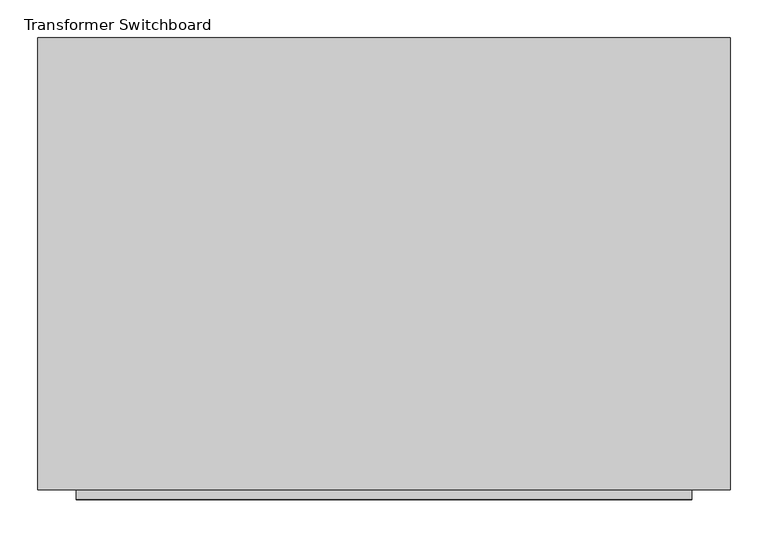
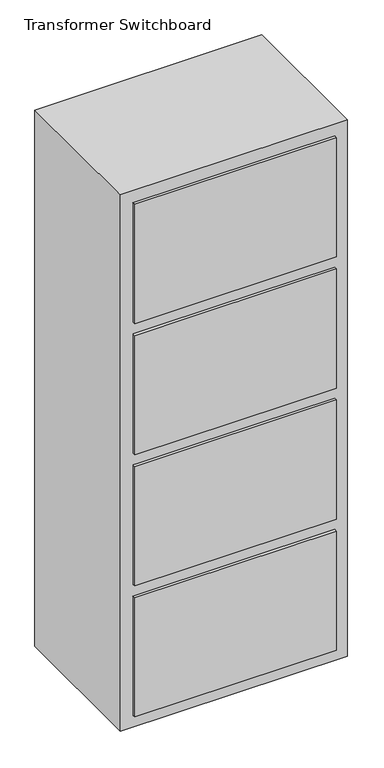
"""IFC4 building model written with IfcOpenShell, lengths in millimetres: proxy geometry, Transformer Switchboard."""

import ifcopenshell
import ifcopenshell.guid

model = None  # the IFC model being written
_history = None  # IfcOwnerHistory: only IFC2X3 demands one
_inside = {}  # id of a spatial element -> (the spatial element, [elements in it])
_under = {}  # id of a project, library or spatial element -> (it, [spatial elements below it])
_declared = {}  # id of a project -> (the project, [libraries it declares])
_typed = {}  # id of a type object -> (the type object, [elements of that type])
_made_of = {}  # id of a material, layer set ... -> (it, [elements and type objects made of it])


def new_model(schema):
    """Start an empty IFC model of exactly this schema.

    Asked for "IFC4X3", IfcOpenShell would pick the latest addendum, in which some entities
    have other attributes; the version numbers below select the first issue.
    IFC2X3 requires an IfcOwnerHistory on every rooted entity: one is made here for all.
    """
    global model, _history
    if schema == "IFC4X3":
        model = ifcopenshell.file(schema_version=(4, 3, 0, 0))
    else:
        model = ifcopenshell.file(schema=schema)
    _inside.clear()
    _under.clear()
    _declared.clear()
    _typed.clear()
    _made_of.clear()
    _history = None
    if model.schema == "IFC2X3":
        org = make("IfcOrganization", Name="unknown")
        user = make(
            "IfcPersonAndOrganization",
            ThePerson=make("IfcPerson", FamilyName="unknown"),
            TheOrganization=org,
        )
        app = make(
            "IfcApplication",
            ApplicationDeveloper=org,
            Version="unknown",
            ApplicationFullName="unknown",
            ApplicationIdentifier="unknown",
        )
        _history = make(
            "IfcOwnerHistory",
            OwningUser=user,
            OwningApplication=app,
            ChangeAction="ADDED",
            CreationDate=0,
        )
    return model


def make(cls, **values):
    """One entity of the class cls with the attributes given. An attribute that is None is left unset."""
    return model.create_entity(
        cls, **{name: value for name, value in values.items() if value is not None}
    )


def rooted(cls, **values):
    """An entity with a GlobalId (a new one), such as an element, a storey or a relation."""
    return make(cls, GlobalId=ifcopenshell.guid.new(), OwnerHistory=_history, **values)


def si_unit(unit_type, name, prefix=None):
    """IfcSIUnit, for example si_unit("LENGTHUNIT", "METRE", prefix="MILLI")."""
    return make("IfcSIUnit", UnitType=unit_type, Prefix=prefix, Name=name)


def assignment(units):
    """IfcUnitAssignment: the units of a project."""
    return None if units is None else make("IfcUnitAssignment", Units=units)


def point(xyz):
    """IfcCartesianPoint."""
    return None if xyz is None else make("IfcCartesianPoint", Coordinates=xyz)


def direction(xyz):
    """IfcDirection."""
    return None if xyz is None else make("IfcDirection", DirectionRatios=xyz)


def frame(location, z_axis=None, x_axis=None):
    """IfcAxis2Placement3D, a coordinate frame: its origin and axes. An axis left out is left unset."""
    return make(
        "IfcAxis2Placement3D",
        Location=point(location),
        Axis=direction(z_axis),
        RefDirection=direction(x_axis),
    )


def origin():
    """The frame at (0, 0, 0) with its axes left unset."""
    return frame((0.0, 0.0, 0.0))


def origin_with_axes():
    """The frame at (0, 0, 0) with the z axis (0, 0, 1) and the x axis (1, 0, 0) written out."""
    return frame((0.0, 0.0, 0.0), z_axis=(0.0, 0.0, 1.0), x_axis=(1.0, 0.0, 0.0))


def place(relative_to, where):
    """IfcLocalPlacement: puts the frame where relative to a parent placement (None: the world)."""
    return make(
        "IfcLocalPlacement", PlacementRelTo=relative_to, RelativePlacement=where
    )


def context(
    kind, dimensions, precision=None, world=None, true_north=None, identifier=None
):
    """IfcGeometricRepresentationContext, for example the 3D "Model" context."""
    return make(
        "IfcGeometricRepresentationContext",
        ContextIdentifier=identifier,
        ContextType=kind,
        CoordinateSpaceDimension=dimensions,
        Precision=precision,
        WorldCoordinateSystem=world,
        TrueNorth=true_north,
    )


def project(units=None, contexts=None):
    """IfcProject with its units and contexts."""
    return rooted(
        "IfcProject",
        Name="project",
        RepresentationContexts=contexts,
        UnitsInContext=assignment(units),
    )


def spatial(cls, under=None, at=None, **own):
    """A site, building, storey or space (cls), placed at a placement, below another one or the project."""
    s = rooted(cls, ObjectPlacement=at, **own)
    if under is not None:
        _under.setdefault(under.id(), (under, []))[1].append(s)
    return s


def polyline(points):
    """IfcPolyline through the points."""
    return make("IfcPolyline", Points=[point(p) for p in points])


def outline(outer, holes=None, kind="AREA"):
    """IfcArbitraryClosedProfileDef: a profile drawn as a closed curve; with holes, ...WithVoids."""
    if holes is None:
        return make("IfcArbitraryClosedProfileDef", ProfileType=kind, OuterCurve=outer)
    return make(
        "IfcArbitraryProfileDefWithVoids",
        ProfileType=kind,
        OuterCurve=outer,
        InnerCurves=holes,
    )


def extrude(swept, where, along, depth):
    """IfcExtrudedAreaSolid: the profile swept, set in the frame where, extruded along a direction by depth."""
    return make(
        "IfcExtrudedAreaSolid",
        SweptArea=swept,
        Position=where,
        ExtrudedDirection=direction(along),
        Depth=depth,
    )


def shape(context_of_items, identifier, shape_type, items):
    """IfcShapeRepresentation: the items that make up one representation, for example the "Body"."""
    return make(
        "IfcShapeRepresentation",
        ContextOfItems=context_of_items,
        RepresentationIdentifier=identifier,
        RepresentationType=shape_type,
        Items=items,
    )


def source(mapping_origin, context_of_items, identifier, shape_type, items):
    """IfcRepresentationMap: a shape defined once, which mapped items show again and again."""
    return make(
        "IfcRepresentationMap",
        MappingOrigin=mapping_origin,
        MappedRepresentation=shape(context_of_items, identifier, shape_type, items),
    )


def transform(
    local_origin,
    x_axis=None,
    y_axis=None,
    z_axis=None,
    scale=None,
    scale2=None,
    scale3=None,
    uniform=True,
):
    """IfcCartesianTransformationOperator3D, or its non-uniform kind. x_axis, y_axis, z_axis: its Axis1, 2, 3."""
    if uniform:
        return make(
            "IfcCartesianTransformationOperator3D",
            Axis1=direction(x_axis),
            Axis2=direction(y_axis),
            LocalOrigin=point(local_origin),
            Scale=scale,
            Axis3=direction(z_axis),
        )
    return make(
        "IfcCartesianTransformationOperator3DnonUniform",
        Axis1=direction(x_axis),
        Axis2=direction(y_axis),
        LocalOrigin=point(local_origin),
        Scale=scale,
        Axis3=direction(z_axis),
        Scale2=scale2,
        Scale3=scale3,
    )


def mapped(mapping_source, mapping_target):
    """IfcMappedItem: shows the shape of a source again, moved by a transform."""
    return make(
        "IfcMappedItem", MappingSource=mapping_source, MappingTarget=mapping_target
    )


def made_of(thing, what):
    """Note that an element or type object is made of a material, layer set ...; save() writes the relation."""
    if what is not None:
        _made_of.setdefault(what.id(), (what, []))[1].append(thing)
    return thing


def element(
    cls,
    number,
    at=None,
    inside=None,
    cuts=None,
    type_object=None,
    material=None,
    context=None,
    identifier="Body",
    shape_type=None,
    held_by="IfcProductDefinitionShape",
    body=None,
    shapes=None,
    **own,
):
    """One element of the class cls, such as IfcWall. Its Tag is "e" and its number.

    at: its placement. inside: the storey or other place that contains it. cuts: it is an
    opening in that element (IfcRelVoidsElement). A single representation is given by context,
    identifier, shape_type and body (its items); several are given by shapes. held_by: the class
    of the entity that holds the representations. save() writes the other relations.
    """
    e = rooted(cls, Tag="e%d" % number, ObjectPlacement=at, **own)
    if body is not None:
        shapes = [shape(context, identifier, shape_type, body)]
    if shapes is not None:
        e.Representation = make(held_by, Representations=shapes)
    if inside is not None:
        _inside.setdefault(inside.id(), (inside, []))[1].append(e)
    if cuts is not None:
        rooted(
            "IfcRelVoidsElement", RelatingBuildingElement=cuts, RelatedOpeningElement=e
        )
    if type_object is not None:
        _typed.setdefault(type_object.id(), (type_object, []))[1].append(e)
    return made_of(e, material)


def aggregate(whole, parts):
    """IfcRelAggregates: a whole, such as a stair, and the parts it consists of."""
    return rooted("IfcRelAggregates", RelatingObject=whole, RelatedObjects=parts)


def save(model, path):
    """Write the relations noted so far, then the file.

    IfcRelAggregates (storeys below a building ...), IfcRelContainedInSpatialStructure (elements
    in a storey), IfcRelDefinesByType, IfcRelAssociatesMaterial and IfcRelDeclares: one each for
    every whole, place, type object, material and project.
    """
    for whole, parts in _under.values():
        aggregate(whole, parts)
    for where, things in _inside.values():
        rooted(
            "IfcRelContainedInSpatialStructure",
            RelatedElements=things,
            RelatingStructure=where,
        )
    for kind, things in _typed.values():
        rooted("IfcRelDefinesByType", RelatedObjects=things, RelatingType=kind)
    for what, things in _made_of.values():
        rooted("IfcRelAssociatesMaterial", RelatedObjects=things, RelatingMaterial=what)
    for by, libraries in _declared.values():
        rooted("IfcRelDeclares", RelatingContext=by, RelatedDefinitions=libraries)
    model.write(path)


def transformer_switchboard_ad6aeb5d(model_context):
    return source(origin(), model_context, "Body", "SweptSolid", [
        extrude(outline(polyline([(406.4, -609.6), (-406.4, -609.6), (-406.4, -596.9), (406.4, -596.9), (406.4, -609.6)])), frame((0.0, 0.0, 1727.2), z_axis=(0.0, 0.0, 1.0), x_axis=(1.0, 0.0, 0.0)), (0.0, 0.0, 1.0), 508.0),
        extrude(outline(polyline([(406.4, -609.6), (-406.4, -609.6), (-406.4, -596.9), (406.4, -596.9), (406.4, -609.6)])), frame((0.0, 0.0, 1168.4), z_axis=(0.0, 0.0, 1.0), x_axis=(1.0, 0.0, 0.0)), (0.0, 0.0, 1.0), 508.0),
        extrude(outline(polyline([(406.4, -609.6), (-406.4, -609.6), (-406.4, -596.9), (406.4, -596.9), (406.4, -609.6)])), frame((0.0, 0.0, 609.6), z_axis=(0.0, 0.0, 1.0), x_axis=(1.0, 0.0, 0.0)), (0.0, 0.0, 1.0), 508.0),
        extrude(outline(polyline([(406.4, -609.6), (-406.4, -609.6), (-406.4, -596.9), (406.4, -596.9), (406.4, -609.6)])), frame((0.0, 0.0, 50.8), z_axis=(0.0, 0.0, 1.0), x_axis=(1.0, 0.0, 0.0)), (0.0, 0.0, 1.0), 508.0),
        extrude(outline(polyline([(457.2, 0.0), (457.2, -596.9), (-457.2, -596.9), (-457.2, 0.0), (457.2, 0.0)])), origin_with_axes(), (0.0, 0.0, 1.0), 2286.0),
    ])


if __name__ == "__main__":
    model = new_model("IFC4")
    model_context = context("Model", 3, world=origin())
    ifc_project = project(units=[si_unit("LENGTHUNIT", "METRE", prefix="MILLI")], contexts=[model_context])
    site = spatial("IfcSite", under=ifc_project)
    building = spatial("IfcBuilding", under=site)
    placement = place(None, origin())
    transformer_switchboard_shape = transformer_switchboard_ad6aeb5d(model_context)
    element("IfcBuildingElementProxy", 1, Name="Transformer Switchboard : 24\"deep x 36\" wide x 90\"H", ObjectType="Transformer Switchboard : 24\"deep x 36\" wide x 90\"H", at=placement, inside=building, context=model_context, shape_type="MappedRepresentation", body=[
        mapped(transformer_switchboard_shape, transform((0.0, 0.0, 0.0), x_axis=(1.0, 0.0, 0.0), y_axis=(0.0, 1.0, 0.0), z_axis=(0.0, 0.0, 1.0))),
    ])
    save(model, "model.ifc")

# Revit data of these elements
# Type "Transformer Switchboard : 24\"deep x 36\" wide x 90\"H"
#   Type Mark = "SG-1"
#   Switchboard Width = 2' - 0"
#   Switchboard Length = 3' - 0"
#   Switchboard Height = 7' - 6"
#   Primary Voltage = 480 V
#   Panel Length = 2' - 8"
#   Panel Height = 1' - 8"
#   Length 1 = 3' - 0"
#   Height 1 = 7' - 6"
#   Half Switchboard Length = 1' - 6"
#   Clearance_Side_Back = 2' - 0"
#   Clearance_Front = 5' - 0"
#   Primary Number of Poles = 3
#   Switchboard Material = none
#   Load Classification = Other
